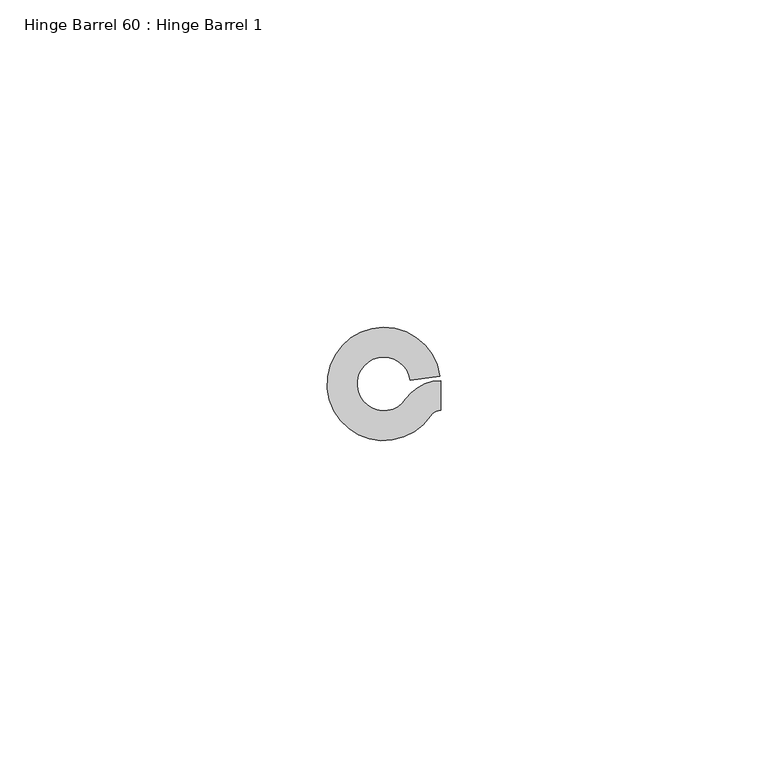
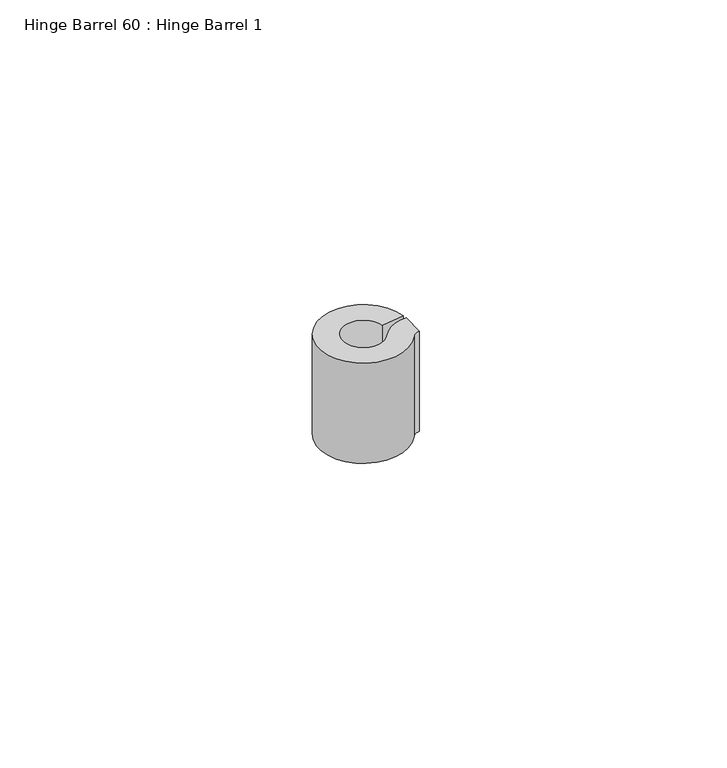
"""IFC4 building model written with IfcOpenShell, lengths in millimetres: proxy geometry, Hinge Barrel 60 : Hinge Barrel 1."""

from ifc_helpers import new_model, si_unit, point, frame, frame_2d, origin, place, context, project, spatial, polyline, circle_curve, trimmed, segment, composite_curve, outline, extrude, source, transform, mapped, element, save


def hinge_barrel_60_hinge_barrel_1_fe703ea2(model_context):
    return source(origin(), model_context, "Body", "SweptSolid", [
        extrude(outline(composite_curve([segment(trimmed(circle_curve(frame_2d((587327.8245257, -536316.2443067)), 6.4044851), [point((587322.5194669, -536312.6563017))], [point((587327.8245257, -536309.8398216))], False, "CARTESIAN"), True, "CONTINUOUS"), segment(polyline([(587327.8245257, -536309.8398216), (587327.8245257, -536314.4038841)]), True, "CONTINUOUS"), segment(trimmed(circle_curve(frame_2d((587327.8245257, -536316.2443067)), 1.8404226), [point((587327.8245257, -536314.4038841))], [point((587326.3000393, -536315.2132409))], True, "CARTESIAN"), True, "CONTINUOUS"), segment(trimmed(circle_curve(frame_2d((587319.1320739, -536310.3652841)), 8.6534625), [point((587326.3000393, -536315.2132409))], [point((587327.7022899, -536309.1678654))], False, "CARTESIAN"), True, "CONTINUOUS"), segment(polyline([(587327.7022899, -536309.1678654), (587323.1821338, -536309.7994153)]), True, "CONTINUOUS"), segment(trimmed(circle_curve(frame_2d((587319.1320739, -536310.3652841)), 4.0894), [point((587323.1821338, -536309.7994153))], [point((587322.5194669, -536312.6563017))], True, "CARTESIAN"), True, "CONTINUOUS")], self_intersect=False)), frame((0.0, 0.0, 438.15), z_axis=(0.0, 0.0, 1.0), x_axis=(1.0, 0.0, 0.0)), (0.0, 0.0, 1.0), 20.8359375),
    ])


if __name__ == "__main__":
    model = new_model("IFC4")
    model_context = context("Model", 3, world=origin())
    ifc_project = project(units=[si_unit("LENGTHUNIT", "METRE", prefix="MILLI")], contexts=[model_context])
    site = spatial("IfcSite", under=ifc_project)
    building = spatial("IfcBuilding", under=site)
    placement = place(None, origin())
    hinge_barrel_60_hinge_barrel_1_shape = hinge_barrel_60_hinge_barrel_1_fe703ea2(model_context)
    element("IfcBuildingElementProxy", 1, Name="Hinge Barrel 60 : Hinge Barrel 1", ObjectType="Hinge Barrel 60 : Hinge Barrel 1", at=placement, inside=building, context=model_context, shape_type="MappedRepresentation", body=[
        mapped(hinge_barrel_60_hinge_barrel_1_shape, transform((0.0, 0.0, 0.0), x_axis=(1.0, 0.0, 0.0), y_axis=(0.0, 1.0, 0.0), z_axis=(0.0, 0.0, 1.0))),
    ])
    save(model, "model.ifc")

# Revit data of these elements
# Element 1 (IfcBuildingElementProxy, "Hinge Barrel 60 : Hinge Barrel 1")
#   Materials on its faces: "6\"X6\" WELD-ON STL BUTT HINGE"
# Materials
#   "6\"X6\" WELD-ON STL BUTT HINGE": class "Metal", colour RGB 189 187 185, transparency 0, Description = "Carbon steel", Cost = 0
